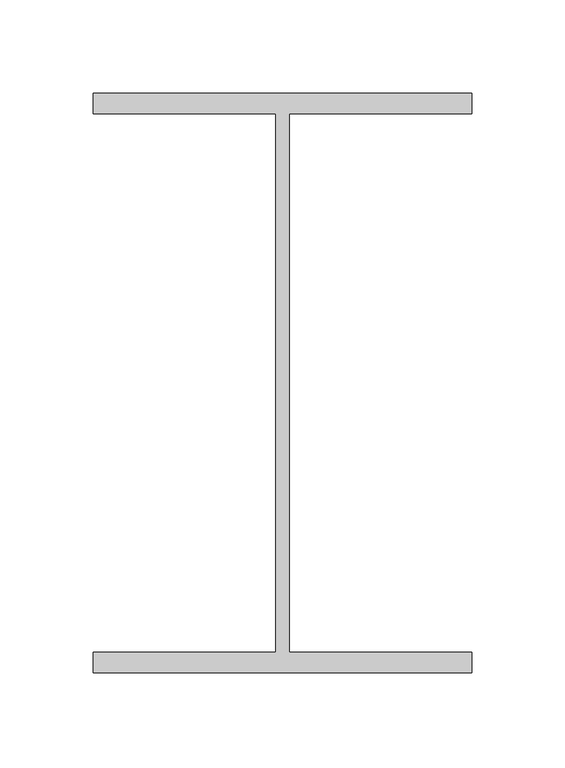
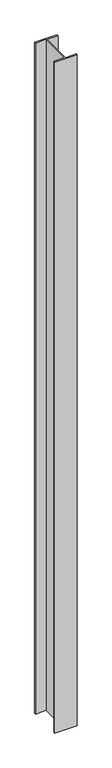
"""IFC4 building model written with IfcOpenShell, lengths in millimetres: proxy geometry, Generic Models 2:Generic Models 2:310765:Generic Models 2:310765 : Generic Models 2:Generic Models 2:310765:57 : Generic Models 2:Generic Models 2:310765:Generic Models 2:310765 : Generic Models 2:Generic Models 2:310765:300385."""

from ifc_helpers import new_model, si_unit, frame, origin, place, context, project, spatial, polyline, outline, extrude, source, transform, mapped, element, save


def generic_models_cb1837ad(model_context):
    return source(origin(), model_context, "Body", "SweptSolid", [
        extrude(outline(polyline([(579104.5117239, -567621.4913841), (579104.5117239, -567632.5046653), (579006.5828177, -567632.5046653), (579006.5828177, -567921.6281028), (579104.5117239, -567921.6281028), (579104.5117239, -567932.6413841), (578901.2863239, -567932.6413841), (578901.2863239, -567921.6281028), (578999.2406302, -567921.6281028), (578999.2406302, -567632.5046653), (578901.3117239, -567632.5046653), (578901.3117239, -567621.4913841), (579104.5117239, -567621.4913841)])), frame((0.0, 0.0, -279.1590326), z_axis=(0.0, 0.0, 1.0), x_axis=(1.0, 0.0, 0.0)), (0.0, 0.0, 1.0), 6413.2590326),
    ])


if __name__ == "__main__":
    model = new_model("IFC4")
    model_context = context("Model", 3, world=origin())
    ifc_project = project(units=[si_unit("LENGTHUNIT", "METRE", prefix="MILLI")], contexts=[model_context])
    site = spatial("IfcSite", under=ifc_project)
    building = spatial("IfcBuilding", under=site)
    placement = place(None, origin())
    generic_models_shape = generic_models_cb1837ad(model_context)
    element("IfcBuildingElementProxy", 1, Name="Generic Models 2:Generic Models 2:310765:Generic Models 2:310765 : Generic Models 2:Generic Models 2:310765:57 : Generic Models 2:Generic Models 2:310765:Generic Models 2:310765 : Generic Models 2:Generic Models 2:310765:300385", ObjectType="Generic Models 2:Generic Models 2:310765:Generic Models 2:310765 : Generic Models 2:Generic Models 2:310765:57 : Generic Models 2:Generic Models 2:310765:Generic Models 2:310765 : Generic Models 2:Generic Models 2:310765:300385", at=placement, inside=building, context=model_context, shape_type="MappedRepresentation", body=[
        mapped(generic_models_shape, transform((0.0, 0.0, 0.0), x_axis=(1.0, 0.0, 0.0), y_axis=(0.0, 1.0, 0.0), z_axis=(0.0, 0.0, 1.0))),
    ])
    save(model, "model.ifc")

# Revit data of these elements
# Type "Generic Models 2:Generic Models 2:310765:Generic Models 2:310765 : Generic Models 2:Generic Models 2:310765:57 : Generic Models 2:Generic Models 2:310765:Generic Models 2:310765 : Generic Models 2:Generic Models 2:310765:300385"
#   NameOverride = "Generic Models 2:Generic Models 2:310765:Generic Models 2:310765 : Generic Models 2:Generic Models 2:310765:300385"
#   ObjectTypeOverride = "Generic Models 2:310765 : Generic Models 2:Generic Models 2:310765"
#   Reference = "Generic Models 2"
#   Tag = "300385"
# Element 1 (IfcBuildingElementProxy, "Generic Models 2:Generic Models 2:310765:Generic Models 2:310765 : Generic Models 2:Generic Models 2:310765:57 : Generic Models 2:Generic Models 2:310765:Generic Models 2:310765 : Generic Models 2:Generic Models 2:310765:300385")
#   Materials on its faces: "STRUCTURAL STEEL - SEE STRUCT. DWGS"
# Materials
#   "STRUCTURAL STEEL - SEE STRUCT. DWGS": class "Metal", colour RGB 189 187 185, transparency 0, Description = "Structural steel 50ksi", Cost = 0
